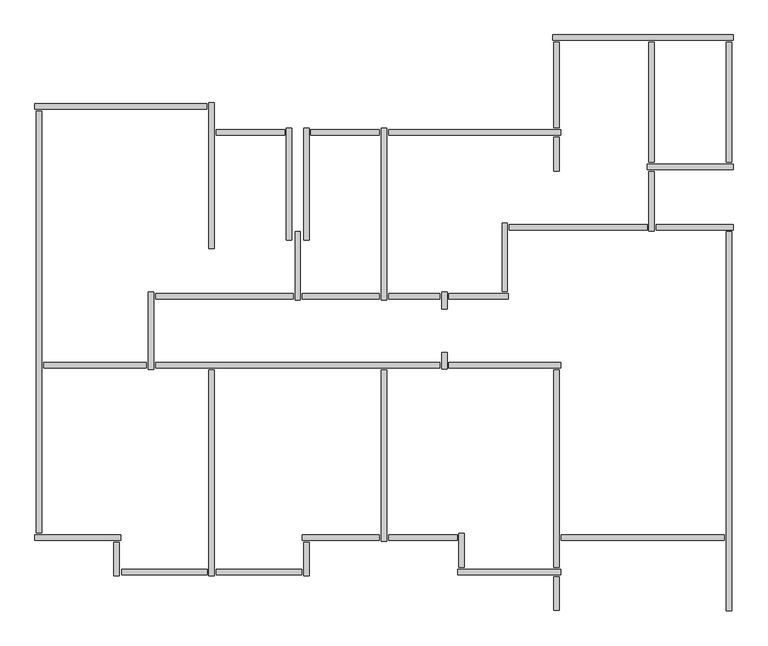
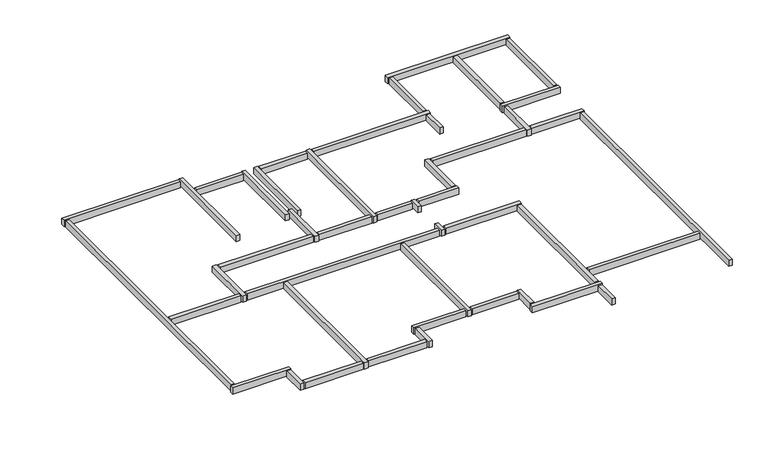
"""IFC4 building model written with IfcOpenShell, lengths in millimetres: beam geometry, Graute viga de respaldo10 : Graute viga de respaldo."""

from ifc_helpers import new_model, si_unit, frame, origin, place, context, project, spatial, polyline, outline, extrude, source, transform, mapped, element, save


def beam_af594a03(model_context):
    return source(origin(), model_context, "Body", "SweptSolid", [
        extrude(outline(polyline([(-75401.7587292, 57502.4278788), (-75401.7587292, 57408.4278788), (-76591.7587292, 57408.4278788), (-76591.7587292, 57502.4278788), (-75401.7587292, 57502.4278788)])), frame((0.0, 0.0, 8632.9999999), z_axis=(0.0, 0.0, 1.0), x_axis=(1.0, 0.0, 0.0)), (0.0, 0.0, 1.0), 167.0),
        extrude(outline(polyline([(-73751.7587292, 57502.4278788), (-73751.7587292, 57408.4278788), (-74941.7587292, 57408.4278788), (-74941.7587292, 57502.4278788), (-73751.7587292, 57502.4278788)])), frame((0.0, 0.0, 8632.9999999), z_axis=(0.0, 0.0, 1.0), x_axis=(1.0, 0.0, 0.0)), (0.0, 0.0, 1.0), 167.0),
        extrude(outline(polyline([(-77801.7587292, 53452.4278788), (-77801.7587292, 53358.4278788), (-79591.7587292, 53358.4278788), (-79591.7587292, 53452.4278788), (-77801.7587292, 53452.4278788)])), frame((0.0, 0.0, 8632.9999999), z_axis=(0.0, 0.0, 1.0), x_axis=(1.0, 0.0, 0.0)), (0.0, 0.0, 1.0), 167.0),
        extrude(outline(polyline([(-72401.7587292, 50452.4278788), (-72401.7587292, 50358.4278788), (-73591.7587292, 50358.4278788), (-73591.7587292, 50452.4278788), (-72401.7587292, 50452.4278788)])), frame((0.0, 0.0, 8632.9999999), z_axis=(0.0, 0.0, 1.0), x_axis=(1.0, 0.0, 0.0)), (0.0, 0.0, 1.0), 167.0),
        extrude(outline(polyline([(-72368.7587292, 50475.4278788), (-72274.7587292, 50475.4278788), (-72274.7587292, 49885.4278788), (-72368.7587292, 49885.4278788), (-72368.7587292, 50475.4278788)])), frame((0.0, 0.0, 8632.9999999), z_axis=(0.0, 0.0, 1.0), x_axis=(1.0, 0.0, 0.0)), (0.0, 0.0, 1.0), 167.0),
        extrude(outline(polyline([(-70601.7587292, 49852.4278788), (-70601.7587292, 49758.4278788), (-72391.7587292, 49758.4278788), (-72391.7587292, 49852.4278788), (-70601.7587292, 49852.4278788)])), frame((0.0, 0.0, 8632.9999999), z_axis=(0.0, 0.0, 1.0), x_axis=(1.0, 0.0, 0.0)), (0.0, 0.0, 1.0), 167.0),
        extrude(outline(polyline([(-72574.7587292, 53335.4278788), (-72668.7587292, 53335.4278788), (-72668.7587292, 53625.4278788), (-72574.7587292, 53625.4278788), (-72574.7587292, 53335.4278788)])), frame((0.0, 0.0, 8632.9999999), z_axis=(0.0, 0.0, 1.0), x_axis=(1.0, 0.0, 0.0)), (0.0, 0.0, 1.0), 167.0),
        extrude(outline(polyline([(-75251.7587292, 54652.4278788), (-75251.7587292, 54558.4278788), (-77641.7587292, 54558.4278788), (-77641.7587292, 54652.4278788), (-75251.7587292, 54652.4278788)])), frame((0.0, 0.0, 8632.9999999), z_axis=(0.0, 0.0, 1.0), x_axis=(1.0, 0.0, 0.0)), (0.0, 0.0, 1.0), 167.0),
        extrude(outline(polyline([(-73751.7587292, 54652.4278788), (-73751.7587292, 54558.4278788), (-75091.7587292, 54558.4278788), (-75091.7587292, 54652.4278788), (-73751.7587292, 54652.4278788)])), frame((0.0, 0.0, 8632.9999999), z_axis=(0.0, 0.0, 1.0), x_axis=(1.0, 0.0, 0.0)), (0.0, 0.0, 1.0), 167.0),
        extrude(outline(polyline([(-72701.7587292, 54652.4278788), (-72701.7587292, 54558.4278788), (-73591.7587292, 54558.4278788), (-73591.7587292, 54652.4278788), (-72701.7587292, 54652.4278788)])), frame((0.0, 0.0, 8632.9999999), z_axis=(0.0, 0.0, 1.0), x_axis=(1.0, 0.0, 0.0)), (0.0, 0.0, 1.0), 167.0),
        extrude(outline(polyline([(-72574.7587292, 54385.4278788), (-72668.7587292, 54385.4278788), (-72668.7587292, 54675.4278788), (-72574.7587292, 54675.4278788), (-72574.7587292, 54385.4278788)])), frame((0.0, 0.0, 8632.9999999), z_axis=(0.0, 0.0, 1.0), x_axis=(1.0, 0.0, 0.0)), (0.0, 0.0, 1.0), 167.0),
        extrude(outline(polyline([(-71511.7587292, 54652.4278788), (-71511.7587292, 54558.4278788), (-72541.7587292, 54558.4278788), (-72541.7587292, 54652.4278788), (-71511.7587292, 54652.4278788)])), frame((0.0, 0.0, 8632.9999999), z_axis=(0.0, 0.0, 1.0), x_axis=(1.0, 0.0, 0.0)), (0.0, 0.0, 1.0), 167.0),
        extrude(outline(polyline([(-71618.7587292, 55875.4278788), (-71524.7587292, 55875.4278788), (-71524.7587292, 54685.4278788), (-71618.7587292, 54685.4278788), (-71618.7587292, 55875.4278788)])), frame((0.0, 0.0, 8632.9999999), z_axis=(0.0, 0.0, 1.0), x_axis=(1.0, 0.0, 0.0)), (0.0, 0.0, 1.0), 167.0),
        extrude(outline(polyline([(-69091.7587292, 55852.4278788), (-69091.7587292, 55758.4278788), (-71491.7587292, 55758.4278788), (-71491.7587292, 55852.4278788), (-69091.7587292, 55852.4278788)])), frame((0.0, 0.0, 8632.9999999), z_axis=(0.0, 0.0, 1.0), x_axis=(1.0, 0.0, 0.0)), (0.0, 0.0, 1.0), 167.0),
        extrude(outline(polyline([(-73624.7587292, 54540.4278788), (-73718.7587292, 54540.4278788), (-73718.7587292, 57525.4278788), (-73624.7587292, 57525.4278788), (-73624.7587292, 54540.4278788)])), frame((0.0, 0.0, 8632.9999999), z_axis=(0.0, 0.0, 1.0), x_axis=(1.0, 0.0, 0.0)), (0.0, 0.0, 1.0), 167.0),
        extrude(outline(polyline([(-70601.7587292, 57502.4278788), (-70601.7587292, 57408.4278788), (-73591.7587292, 57408.4278788), (-73591.7587292, 57502.4278788), (-70601.7587292, 57502.4278788)])), frame((0.0, 0.0, 8632.9999999), z_axis=(0.0, 0.0, 1.0), x_axis=(1.0, 0.0, 0.0)), (0.0, 0.0, 1.0), 167.0),
        extrude(outline(polyline([(-70624.7587292, 56785.4278788), (-70718.7587292, 56785.4278788), (-70718.7587292, 57375.4278788), (-70624.7587292, 57375.4278788), (-70624.7587292, 56785.4278788)])), frame((0.0, 0.0, 8632.9999999), z_axis=(0.0, 0.0, 1.0), x_axis=(1.0, 0.0, 0.0)), (0.0, 0.0, 1.0), 167.0),
        extrude(outline(polyline([(-70718.7587292, 59025.4278788), (-70624.7587292, 59025.4278788), (-70624.7587292, 57535.4278788), (-70718.7587292, 57535.4278788), (-70718.7587292, 59025.4278788)])), frame((0.0, 0.0, 8632.9999999), z_axis=(0.0, 0.0, 1.0), x_axis=(1.0, 0.0, 0.0)), (0.0, 0.0, 1.0), 167.0),
        extrude(outline(polyline([(-67718.7587292, 59025.4278788), (-67624.7587292, 59025.4278788), (-67624.7587292, 56935.4278788), (-67718.7587292, 56935.4278788), (-67718.7587292, 59025.4278788)])), frame((0.0, 0.0, 8632.9999999), z_axis=(0.0, 0.0, 1.0), x_axis=(1.0, 0.0, 0.0)), (0.0, 0.0, 1.0), 167.0),
        extrude(outline(polyline([(-69068.7587292, 59025.4278788), (-68974.7587292, 59025.4278788), (-68974.7587292, 56935.4278788), (-69068.7587292, 56935.4278788), (-69068.7587292, 59025.4278788)])), frame((0.0, 0.0, 8632.9999999), z_axis=(0.0, 0.0, 1.0), x_axis=(1.0, 0.0, 0.0)), (0.0, 0.0, 1.0), 167.0),
        extrude(outline(polyline([(-68974.7587292, 55735.4278788), (-69068.7587292, 55735.4278788), (-69068.7587292, 56775.4278788), (-68974.7587292, 56775.4278788), (-68974.7587292, 55735.4278788)])), frame((0.0, 0.0, 8632.9999999), z_axis=(0.0, 0.0, 1.0), x_axis=(1.0, 0.0, 0.0)), (0.0, 0.0, 1.0), 167.0),
        extrude(outline(polyline([(-67751.7587292, 50452.4278788), (-67751.7587292, 50358.4278788), (-70591.7587292, 50358.4278788), (-70591.7587292, 50452.4278788), (-67751.7587292, 50452.4278788)])), frame((0.0, 0.0, 8632.9999999), z_axis=(0.0, 0.0, 1.0), x_axis=(1.0, 0.0, 0.0)), (0.0, 0.0, 1.0), 167.0),
        extrude(outline(polyline([(-70718.7587292, 53325.4278788), (-70624.7587292, 53325.4278788), (-70624.7587292, 49885.4278788), (-70718.7587292, 49885.4278788), (-70718.7587292, 53325.4278788)])), frame((0.0, 0.0, 8632.9999999), z_axis=(0.0, 0.0, 1.0), x_axis=(1.0, 0.0, 0.0)), (0.0, 0.0, 1.0), 167.0),
        extrude(outline(polyline([(-70601.7587292, 53452.4278788), (-70601.7587292, 53358.4278788), (-72541.7587292, 53358.4278788), (-72541.7587292, 53452.4278788), (-70601.7587292, 53452.4278788)])), frame((0.0, 0.0, 8632.9999999), z_axis=(0.0, 0.0, 1.0), x_axis=(1.0, 0.0, 0.0)), (0.0, 0.0, 1.0), 167.0),
        extrude(outline(polyline([(-72701.7587292, 53452.4278788), (-72701.7587292, 53358.4278788), (-77641.7587292, 53358.4278788), (-77641.7587292, 53452.4278788), (-72701.7587292, 53452.4278788)])), frame((0.0, 0.0, 8632.9999999), z_axis=(0.0, 0.0, 1.0), x_axis=(1.0, 0.0, 0.0)), (0.0, 0.0, 1.0), 167.0),
        extrude(outline(polyline([(-73624.7587292, 50335.4278788), (-73718.7587292, 50335.4278788), (-73718.7587292, 53325.4278788), (-73624.7587292, 53325.4278788), (-73624.7587292, 50335.4278788)])), frame((0.0, 0.0, 8632.9999999), z_axis=(0.0, 0.0, 1.0), x_axis=(1.0, 0.0, 0.0)), (0.0, 0.0, 1.0), 167.0),
        extrude(outline(polyline([(-75091.7587292, 50358.4278788), (-75091.7587292, 50452.4278788), (-73751.7587292, 50452.4278788), (-73751.7587292, 50358.4278788), (-75091.7587292, 50358.4278788)])), frame((0.0, 0.0, 8632.9999999), z_axis=(0.0, 0.0, 1.0), x_axis=(1.0, 0.0, 0.0)), (0.0, 0.0, 1.0), 167.0),
        extrude(outline(polyline([(-74974.7587292, 49735.4278788), (-75068.7587292, 49735.4278788), (-75068.7587292, 50325.4278788), (-74974.7587292, 50325.4278788), (-74974.7587292, 49735.4278788)])), frame((0.0, 0.0, 8632.9999999), z_axis=(0.0, 0.0, 1.0), x_axis=(1.0, 0.0, 0.0)), (0.0, 0.0, 1.0), 167.0),
        extrude(outline(polyline([(-75101.7587292, 49852.4278788), (-75101.7587292, 49758.4278788), (-76591.7587292, 49758.4278788), (-76591.7587292, 49852.4278788), (-75101.7587292, 49852.4278788)])), frame((0.0, 0.0, 8632.9999999), z_axis=(0.0, 0.0, 1.0), x_axis=(1.0, 0.0, 0.0)), (0.0, 0.0, 1.0), 167.0),
        extrude(outline(polyline([(-78230.736554, 49758.4278788), (-78230.736554, 49853.4278788), (-76741.7587292, 49853.4278788), (-76741.7587292, 49758.4278788), (-78230.736554, 49758.4278788)])), frame((0.0, 0.0, 8617.1856208), z_axis=(0.0, 0.0, 1.0), x_axis=(1.0, 0.0, 0.0)), (0.0, 0.0, 1.0), 165.0),
        extrude(outline(polyline([(-79718.7587292, 57825.4278788), (-79624.7587292, 57825.4278788), (-79624.7587292, 50485.4278788), (-79718.7587292, 50485.4278788), (-79718.7587292, 57825.4278788)])), frame((0.0, 0.0, 8632.9999999), z_axis=(0.0, 0.0, 1.0), x_axis=(1.0, 0.0, 0.0)), (0.0, 0.0, 1.0), 167.0),
        extrude(outline(polyline([(-77768.7587292, 54675.4278788), (-77674.7587292, 54675.4278788), (-77674.7587292, 53330.0746661), (-77768.7587292, 53330.0746661), (-77768.7587292, 54675.4278788)])), frame((0.0, 0.0, 8632.9999999), z_axis=(0.0, 0.0, 1.0), x_axis=(1.0, 0.0, 0.0)), (0.0, 0.0, 1.0), 167.0),
        extrude(outline(polyline([(-75218.7587292, 55725.4278788), (-75124.7587292, 55725.4278788), (-75124.7587292, 54535.4278788), (-75218.7587292, 54535.4278788), (-75218.7587292, 55725.4278788)])), frame((0.0, 0.0, 8632.9999999), z_axis=(0.0, 0.0, 1.0), x_axis=(1.0, 0.0, 0.0)), (0.0, 0.0, 1.0), 167.0),
        extrude(outline(polyline([(-75368.7587292, 57525.4278788), (-75274.7587292, 57525.4278788), (-75274.7587292, 55585.4278788), (-75368.7587292, 55585.4278788), (-75368.7587292, 57525.4278788)])), frame((0.0, 0.0, 8632.9999999), z_axis=(0.0, 0.0, 1.0), x_axis=(1.0, 0.0, 0.0)), (0.0, 0.0, 1.0), 167.0),
        extrude(outline(polyline([(-75068.7587292, 57525.4278788), (-74974.7587292, 57525.4278788), (-74974.7587292, 55585.4278788), (-75068.7587292, 55585.4278788), (-75068.7587292, 57525.4278788)])), frame((0.0, 0.0, 8632.9999999), z_axis=(0.0, 0.0, 1.0), x_axis=(1.0, 0.0, 0.0)), (0.0, 0.0, 1.0), 167.0),
        extrude(outline(polyline([(-76718.7587292, 57975.4278788), (-76624.7587292, 57975.4278788), (-76624.7587292, 55435.4278788), (-76718.7587292, 55435.4278788), (-76718.7587292, 57975.4278788)])), frame((0.0, 0.0, 8632.9999999), z_axis=(0.0, 0.0, 1.0), x_axis=(1.0, 0.0, 0.0)), (0.0, 0.0, 1.0), 167.0),
        extrude(outline(polyline([(-79741.7587292, 57858.4278788), (-79741.7587292, 57952.4278788), (-76751.7587292, 57952.4278788), (-76751.7587292, 57858.4278788), (-79741.7587292, 57858.4278788)])), frame((0.0, 0.0, 8632.9999999), z_axis=(0.0, 0.0, 1.0), x_axis=(1.0, 0.0, 0.0)), (0.0, 0.0, 1.0), 167.0),
        extrude(outline(polyline([(-78274.7587292, 49735.4278788), (-78368.7587292, 49735.4278788), (-78368.7587292, 50325.4278788), (-78274.7587292, 50325.4278788), (-78274.7587292, 49735.4278788)])), frame((0.0, 0.0, 8632.9999999), z_axis=(0.0, 0.0, 1.0), x_axis=(1.0, 0.0, 0.0)), (0.0, 0.0, 1.0), 167.0),
        extrude(outline(polyline([(-78251.7587292, 50452.4278788), (-78251.7587292, 50358.4278788), (-79741.7587292, 50358.4278788), (-79741.7587292, 50452.4278788), (-78251.7587292, 50452.4278788)])), frame((0.0, 0.0, 8632.9999999), z_axis=(0.0, 0.0, 1.0), x_axis=(1.0, 0.0, 0.0)), (0.0, 0.0, 1.0), 167.0),
        extrude(outline(polyline([(-76624.7587292, 49735.4278788), (-76718.7587292, 49735.4278788), (-76718.7587292, 53325.4278788), (-76624.7587292, 53325.4278788), (-76624.7587292, 49735.4278788)])), frame((0.0, 0.0, 8632.9999999), z_axis=(0.0, 0.0, 1.0), x_axis=(1.0, 0.0, 0.0)), (0.0, 0.0, 1.0), 167.0),
        extrude(outline(polyline([(-70624.7587292, 49135.4278788), (-70718.7587292, 49135.4278788), (-70718.7587292, 49725.4278788), (-70624.7587292, 49725.4278788), (-70624.7587292, 49135.4278788)])), frame((0.0, 0.0, 8632.9999999), z_axis=(0.0, 0.0, 1.0), x_axis=(1.0, 0.0, 0.0)), (0.0, 0.0, 1.0), 167.0),
        extrude(outline(polyline([(-67601.7587292, 56902.4278788), (-67601.7587292, 56808.4278788), (-69091.7587292, 56808.4278788), (-69091.7587292, 56902.4278788), (-67601.7587292, 56902.4278788)])), frame((0.0, 0.0, 8632.9999999), z_axis=(0.0, 0.0, 1.0), x_axis=(1.0, 0.0, 0.0)), (0.0, 0.0, 1.0), 167.0),
        extrude(outline(polyline([(-67601.7587292, 59152.4278788), (-67601.7587292, 59058.4278788), (-70741.7587292, 59058.4278788), (-70741.7587292, 59152.4278788), (-67601.7587292, 59152.4278788)])), frame((0.0, 0.0, 8632.9999999), z_axis=(0.0, 0.0, 1.0), x_axis=(1.0, 0.0, 0.0)), (0.0, 0.0, 1.0), 167.0),
        extrude(outline(polyline([(-67601.7587292, 55852.4278788), (-67601.7587292, 55758.4278788), (-68941.7587292, 55758.4278788), (-68941.7587292, 55852.4278788), (-67601.7587292, 55852.4278788)])), frame((0.0, 0.0, 8632.9999999), z_axis=(0.0, 0.0, 1.0), x_axis=(1.0, 0.0, 0.0)), (0.0, 0.0, 1.0), 167.0),
        extrude(outline(polyline([(-67624.7587292, 49132.8979841), (-67718.7587292, 49132.8979841), (-67718.7587292, 55725.4278788), (-67624.7587292, 55725.4278788), (-67624.7587292, 49132.8979841)])), frame((0.0, 0.0, 8632.9999999), z_axis=(0.0, 0.0, 1.0), x_axis=(1.0, 0.0, 0.0)), (0.0, 0.0, 1.0), 167.0),
    ])


if __name__ == "__main__":
    model = new_model("IFC4")
    model_context = context("Model", 3, world=origin())
    ifc_project = project(units=[si_unit("LENGTHUNIT", "METRE", prefix="MILLI")], contexts=[model_context])
    site = spatial("IfcSite", under=ifc_project)
    building = spatial("IfcBuilding", under=site)
    placement = place(None, origin())
    beam_shape = beam_af594a03(model_context)
    element("IfcBeam", 1, ObjectType="Graute viga de respaldo10 : Graute viga de respaldo", at=placement, inside=building, context=model_context, shape_type="MappedRepresentation", body=[
        mapped(beam_shape, transform((0.0, 0.0, 0.0), x_axis=(1.0, 0.0, 0.0), y_axis=(0.0, 1.0, 0.0), z_axis=(0.0, 0.0, 1.0))),
    ])
    save(model, "model.ifc")

# Revit data of these elements
# Element 1 (IfcBeam, "Graute viga de respaldo10 : Graute viga de respaldo")
#   Materials on its faces: "Concreto, Faixa de areia/cimento"
# Materials
#   "Concreto, Faixa de areia/cimento": class "Concreto", colour RGB 127 127 127, transparency 0, Description = "Revestimento de laje de concreto", Cost = 0
